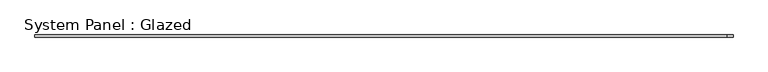
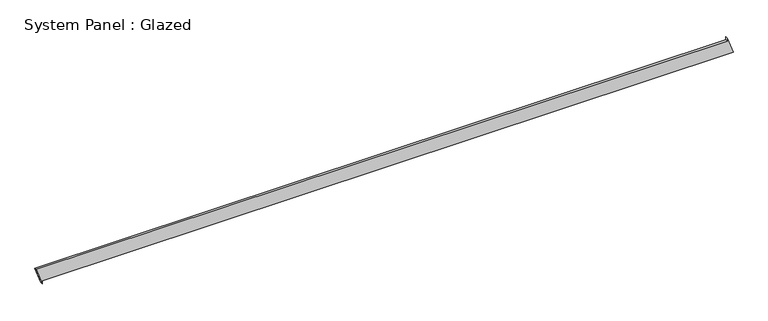
"""IFC4 building model written with IfcOpenShell, lengths in millimetres: plate geometry, System Panel : Glazed."""

from ifc_helpers import new_model, si_unit, frame, origin, place, context, project, spatial, polyline, outline, extrude, source, transform, mapped, element, save


def system_panel_glazed_7537b497(model_context):
    return source(origin(), model_context, "Body", "SweptSolid", [
        extrude(outline(polyline([(0.0, -3959.0229169), (35.3553391, -3959.0229169), (35.3553391, 4028.0764592), (234.64232, 3959.1368322), (199.2869809, 3959.1370419), (199.2396119, -4028.0764592), (0.0, -3959.0229169)])), frame((0.0, -49.5, 0.0), z_axis=(0.0, 1.0, 0.0), x_axis=(0.0, 0.0, 1.0)), (0.0, 0.0, 1.0), 25.0),
    ])


if __name__ == "__main__":
    model = new_model("IFC4")
    model_context = context("Model", 3, world=origin())
    ifc_project = project(units=[si_unit("LENGTHUNIT", "METRE", prefix="MILLI")], contexts=[model_context])
    site = spatial("IfcSite", under=ifc_project)
    building = spatial("IfcBuilding", under=site)
    placement = place(None, origin())
    system_panel_glazed_shape = system_panel_glazed_7537b497(model_context)
    element("IfcPlate", 1, ObjectType="System Panel : Glazed", at=placement, inside=building, context=model_context, shape_type="MappedRepresentation", body=[
        mapped(system_panel_glazed_shape, transform((0.0, 0.0, 0.0), x_axis=(1.0, 0.0, 0.0), y_axis=(0.0, 1.0, 0.0), z_axis=(0.0, 0.0, 1.0))),
    ])
    save(model, "model.ifc")

# Revit data of these elements
# Element 1 (IfcPlate, "System Panel : Glazed")
#   Materials on its faces: "Glass"
# Materials
#   "Glass": class "Glass", colour RGB 218 227 224, transparency 0.85, Description = "Soda Lime Glass", Cost = 0
